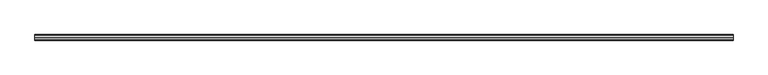
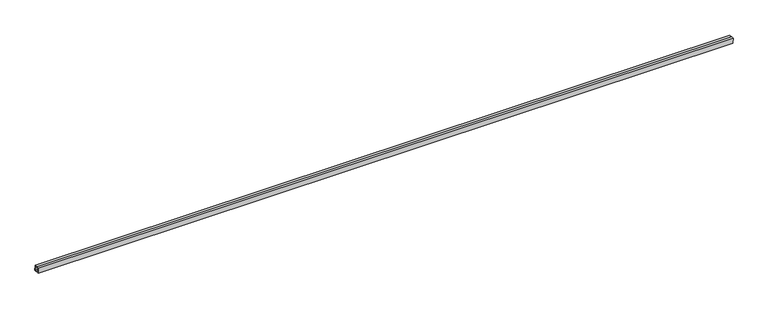
"""IFC4 building model written with IfcOpenShell, lengths in millimetres: proxy geometry, Inner panel:Inner panel:1:Inner panel:1 : Inner panel:Inner panel:300324:2:Inner panel:1:Inner panel:1 : Inner panel:Inner panel:300324:2 : Inner panel:Inner panel:1:Inner panel:1 : Inner panel:Inner panel:300324:300043:16 : Inner panel:Inner panel:1:Inner panel:1 : Inner panel:Inner panel:300324:2:Inner panel:1:Inner panel:1 : Inner panel:Inner panel:300324:2 : Inner panel:Inner panel:1:Inner panel:1 : Inner panel:Inner panel:300324:300043:308120."""

from ifc_helpers import new_model, si_unit, frame, origin, place, context, project, spatial, polyline, outline, extrude, source, transform, mapped, element, save


def generic_models_1d92d81b(model_context):
    return source(origin(), model_context, "Body", "SweptSolid", [
        extrude(outline(polyline([(-576655.6949211, 4047.6065374), (-576637.4544979, 4048.3665551), (-576635.8683742, 4010.299585), (-576673.9353442, 4008.7134612), (-576675.521468, 4046.7804313), (-576657.2810448, 4047.540449), (-576657.1819121, 4045.1612633), (-576673.0431496, 4044.5003784), (-576671.6552914, 4011.1917796), (-576638.3466925, 4012.5796379), (-576639.7345508, 4045.8882367), (-576655.5957883, 4045.2273518), (-576655.6949211, 4047.6065374)])), frame((588245.3367239, 0.0, 0.0), z_axis=(1.0, 0.0, 0.0), x_axis=(0.0, 1.0, 0.0)), (0.0, 0.0, 1.0), 4876.8),
    ])


if __name__ == "__main__":
    model = new_model("IFC4")
    model_context = context("Model", 3, world=origin())
    ifc_project = project(units=[si_unit("LENGTHUNIT", "METRE", prefix="MILLI")], contexts=[model_context])
    site = spatial("IfcSite", under=ifc_project)
    building = spatial("IfcBuilding", under=site)
    placement = place(None, origin())
    generic_models_shape = generic_models_1d92d81b(model_context)
    element("IfcBuildingElementProxy", 1, Name="Inner panel:Inner panel:1:Inner panel:1 : Inner panel:Inner panel:300324:2:Inner panel:1:Inner panel:1 : Inner panel:Inner panel:300324:2 : Inner panel:Inner panel:1:Inner panel:1 : Inner panel:Inner panel:300324:300043:16 : Inner panel:Inner panel:1:Inner panel:1 : Inner panel:Inner panel:300324:2:Inner panel:1:Inner panel:1 : Inner panel:Inner panel:300324:2 : Inner panel:Inner panel:1:Inner panel:1 : Inner panel:Inner panel:300324:300043:308120", ObjectType="Inner panel:Inner panel:1:Inner panel:1 : Inner panel:Inner panel:300324:2:Inner panel:1:Inner panel:1 : Inner panel:Inner panel:300324:2 : Inner panel:Inner panel:1:Inner panel:1 : Inner panel:Inner panel:300324:300043:16 : Inner panel:Inner panel:1:Inner panel:1 : Inner panel:Inner panel:300324:2:Inner panel:1:Inner panel:1 : Inner panel:Inner panel:300324:2 : Inner panel:Inner panel:1:Inner panel:1 : Inner panel:Inner panel:300324:300043:308120", at=placement, inside=building, context=model_context, shape_type="MappedRepresentation", body=[
        mapped(generic_models_shape, transform((0.0, 0.0, 0.0), x_axis=(1.0, 0.0, 0.0), y_axis=(0.0, 1.0, 0.0), z_axis=(0.0, 0.0, 1.0))),
    ])
    save(model, "model.ifc")

# Revit data of these elements
# Type "Inner panel:Inner panel:1:Inner panel:1 : Inner panel:Inner panel:300324:2:Inner panel:1:Inner panel:1 : Inner panel:Inner panel:300324:2 : Inner panel:Inner panel:1:Inner panel:1 : Inner panel:Inner panel:300324:300043:16 : Inner panel:Inner panel:1:Inner panel:1 : Inner panel:Inner panel:300324:2:Inner panel:1:Inner panel:1 : Inner panel:Inner panel:300324:2 : Inner panel:Inner panel:1:Inner panel:1 : Inner panel:Inner panel:300324:300043:308120"
#   NameOverride = "Inner panel:Inner panel:1:Inner panel:1 : Inner panel:Inner panel:300324:2:Inner panel:1:Inner panel:1 : Inner panel:Inner panel:300324:2 : Inner panel:Inner panel:1:Inner panel:1 : Inner panel:Inner panel:300324:300043:308120"
#   ObjectTypeOverride = "Inner panel:1:Inner panel:1 : Inner panel:Inner panel:300324:2 : Inner panel:Inner panel:1:Inner panel:1 : Inner panel:Inner panel:300324:300043"
#   Reference = "Inner panel"
#   Tag = "308120"
# Element 1 (IfcBuildingElementProxy, "Inner panel:Inner panel:1:Inner panel:1 : Inner panel:Inner panel:300324:2:Inner panel:1:Inner panel:1 : Inner panel:Inner panel:300324:2 : Inner panel:Inner panel:1:Inner panel:1 : Inner panel:Inner panel:300324:300043:16 : Inner panel:Inner panel:1:Inner panel:1 : Inner panel:Inner panel:300324:2:Inner panel:1:Inner panel:1 : Inner panel:Inner panel:300324:2 : Inner panel:Inner panel:1:Inner panel:1 : Inner panel:Inner panel:300324:300043:308120")
#   Materials on its faces: "1 1/2\" X 1 1/2\" SPLIT-SEAM SQUARE TUBING (~24\" CANTILEVER FROM C.L. OF GLULAM)"
# Materials
#   "1 1/2\" X 1 1/2\" SPLIT-SEAM SQUARE TUBING (~24\" CANTILEVER FROM C.L. OF GLULAM)": class "Unassigned", colour RGB 202 201 200, transparency 0, Cost = 0
